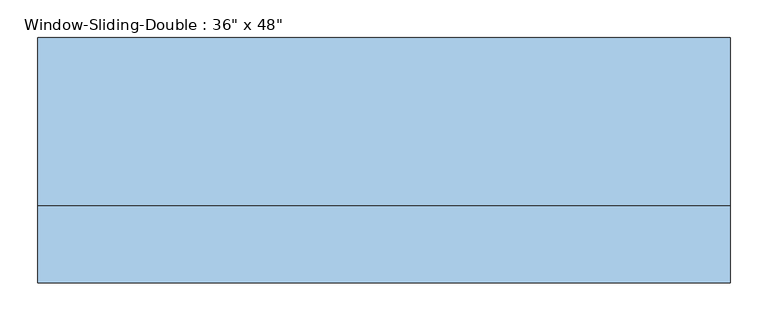
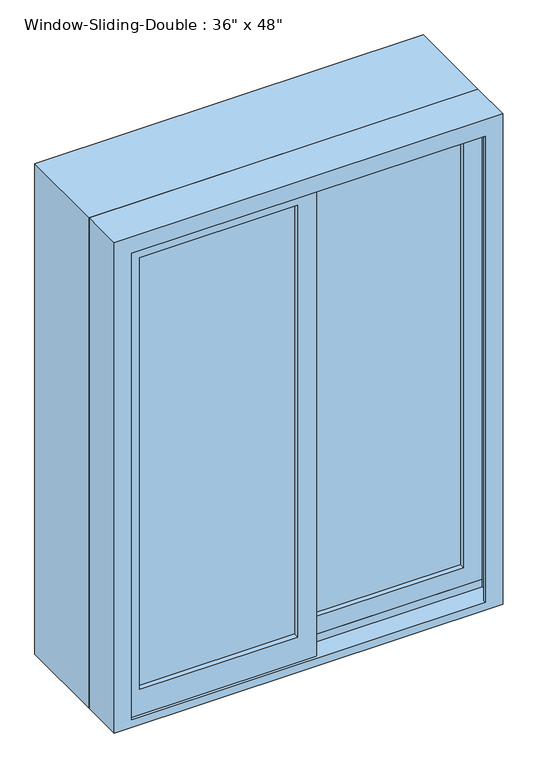
"""IFC4 building model written with IfcOpenShell, lengths in millimetres: window geometry."""

from ifc_helpers import new_model, si_unit, frame, origin, place, context, project, spatial, polyline, outline, extrude, faceted_brep, source, transform, mapped, element, save


def window_970b94cb(model_context):
    return source(origin(), model_context, "Body", "SolidModel", [
        faceted_brep([(-457.2, -66.04, 914.4), (457.2, -66.04, 914.4), (457.2, -167.64, 914.4), (-457.2, -167.64, 914.4), (-416.2778905, -167.64, 2092.6778905), (-416.2778905, -167.64, 933.45), (-416.2778905, -161.29, 933.45), (-416.2778905, -161.29, 2092.6778905), (-438.15, -161.29, 933.45), (-438.15, -161.29, 2114.55), (438.15, -161.29, 2114.55), (438.15, -161.29, 933.45), (416.2778905, -161.29, 933.45), (416.2778905, -161.29, 2092.6778905), (-438.15, -116.84, 933.45), (-438.15, -116.84, 952.5), (-438.15, -72.39, 952.5), (-438.15, -72.39, 933.45), (-438.15, -66.04, 933.45), (-438.15, -66.04, 2114.55), (-457.2, -66.04, 2133.6), (457.2, -66.04, 2133.6), (438.15, -66.04, 2114.55), (438.15, -66.04, 933.45), (-457.2, -167.64, 2133.6), (457.2, -167.64, 2133.6), (416.2778905, -167.64, 2092.6778905), (416.2778905, -167.64, 933.45), (438.15, -72.39, 933.45), (438.15, -72.39, 952.5), (438.15, -116.84, 952.5), (438.15, -116.84, 933.45)], [[[0, 1, 2, 3]], [[4, 5, 6, 7]], [[7, 6, 8, 9, 10, 11, 12, 13]], [[9, 8, 14, 15, 16, 17, 18, 19]], [[0, 20, 21, 1], [22, 19, 18, 23]], [[24, 20, 0, 3]], [[2, 25, 24, 3], [4, 26, 27, 5]], [[7, 13, 26, 4]], [[9, 19, 22, 10]], [[20, 24, 25, 21]], [[13, 12, 27, 26]], [[22, 23, 28, 29, 30, 31, 11, 10]], [[21, 25, 2, 1]], [[27, 12, 11, 31, 14, 8, 6, 5]], [[31, 30, 15, 14]], [[30, 29, 16, 15]], [[29, 28, 17, 16]], [[18, 17, 28, 23]]]),
        extrude(outline(polyline([(2133.6, 457.2), (2133.6, -457.2), (914.4, -457.2), (914.4, 457.2), (2133.6, 457.2)]), holes=[polyline([(2114.55, -438.15), (2114.55, 438.15), (933.45, 438.15), (933.45, -438.15), (2114.55, -438.15)])]), frame((0.0, -66.04, 0.0), z_axis=(0.0, 1.0, 0.0), x_axis=(0.0, 0.0, 1.0)), (0.0, 0.0, 1.0), 222.25),
        extrude(outline(polyline([(393.7, -104.14), (22.225, -104.14), (22.225, -97.79), (393.7, -97.79), (393.7, -104.14)])), frame((0.0, 0.0, 996.95), z_axis=(0.0, 0.0, 1.0), x_axis=(1.0, 0.0, 0.0)), (0.0, 0.0, 1.0), 1073.15),
        extrude(outline(polyline([(393.7, -91.44), (22.225, -91.44), (22.225, -85.09), (393.7, -85.09), (393.7, -91.44)])), frame((0.0, 0.0, 996.95), z_axis=(0.0, 0.0, 1.0), x_axis=(1.0, 0.0, 0.0)), (0.0, 0.0, 1.0), 1073.15),
        extrude(outline(polyline([(-22.225, -148.59), (-393.7, -148.59), (-393.7, -142.24), (-22.225, -142.24), (-22.225, -148.59)])), frame((0.0, 0.0, 996.95), z_axis=(0.0, 0.0, 1.0), x_axis=(1.0, 0.0, 0.0)), (0.0, 0.0, 1.0), 1073.15),
        extrude(outline(polyline([(-22.225, -135.89), (-393.7, -135.89), (-393.7, -129.54), (-22.225, -129.54), (-22.225, -135.89)])), frame((0.0, 0.0, 996.95), z_axis=(0.0, 0.0, 1.0), x_axis=(1.0, 0.0, 0.0)), (0.0, 0.0, 1.0), 1073.15),
        extrude(outline(polyline([(933.45, 22.225), (2114.55, 22.225), (2114.55, -438.15), (933.45, -438.15), (933.45, 22.225)]), holes=[polyline([(2070.1, -393.7), (2070.1, -22.225), (996.95, -22.225), (996.95, -393.7), (2070.1, -393.7)])]), frame((0.0, -161.29, 0.0), z_axis=(0.0, 1.0, 0.0), x_axis=(0.0, 0.0, 1.0)), (0.0, 0.0, 1.0), 44.45),
        extrude(outline(polyline([(952.5, -22.225), (952.5, 438.15), (2114.55, 438.15), (2114.55, -22.225), (952.5, -22.225)]), holes=[polyline([(996.95, 393.7), (996.95, 22.225), (2070.1, 22.225), (2070.1, 393.7), (996.95, 393.7)])]), frame((0.0, -116.84, 0.0), z_axis=(0.0, 1.0, 0.0), x_axis=(0.0, 0.0, 1.0)), (0.0, 0.0, 1.0), 44.45),
    ])


if __name__ == "__main__":
    model = new_model("IFC4")
    model_context = context("Model", 3, world=origin())
    ifc_project = project(units=[si_unit("LENGTHUNIT", "METRE", prefix="MILLI")], contexts=[model_context])
    site = spatial("IfcSite", under=ifc_project)
    building = spatial("IfcBuilding", under=site)
    placement = place(None, origin())
    window_shape = window_970b94cb(model_context)
    element("IfcWindow", 1, ObjectType="Window-Sliding-Double : 36\" x 48\"", at=placement, inside=building, context=model_context, shape_type="MappedRepresentation", body=[
        mapped(window_shape, transform((0.0, 0.0, 0.0), x_axis=(1.0, 0.0, 0.0), y_axis=(0.0, 1.0, 0.0), z_axis=(0.0, 0.0, 1.0))),
    ])
    save(model, "model.ifc")

# Revit data of these elements
# Type "Window-Sliding-Double : 36\" x 48\""
#   Type Mark = "E"
#   Fire Rating = "0.5h"
#   Assembly Code = "B2020100"
#   Analytic Construction = "Double glazing - domestic"
#   Window Inset [instance default] = 0' - 0"
#   Wall Thickness [instance default] = 0' - 6"
#   Visual Light Transmittance = 0.81
#   Thermal Resistance (R) = 1.8146 (h·ft²·°F)/BTU
#   Solar Heat Gain Coefficient = 0.76
#   Muntin Width = 1' - 2 5/8"
#   Muntin Height = 3' - 6 1/4"
#   Interior Wall Closure [instance default] = 0' - 2 3/4"
#   Heat Transfer Coefficient (U) = 0.5511 BTU/(h·ft²·°F)
#   Frame Extension [instance default] = 0' - 0 1/4"
#   Exterior Wall Closure [instance default] = 0' - 1 1/4"
#   Rough Width = 3' - 0 1/2"
#   Rough Height = 4' - 0 1/2"
#   Height = 4' - 0"
#   Extension Jamb [instance default] = 0' - 2 3/4"
#   Default Sill Height = 3' - 0"
#   Width = 3' - 0"
#   Interior Trim Visibility [instance default] = yes
#   Indicator Visibility [instance default] = yes
#   Exterior Trim Visibility [instance default] = yes
#   Muntin Visibility = yes
#   Extension Jamb Visibility [instance default] = yes
#   Muntin Pattern = Muntin Pattern_2x2 : Muntin Pattern_2x2
#   Interior Trim Material = Wood - Stained
#   Interior Trim = Trim-Window-Interior-Flat : Picture Frame
#   Interior Frame Material = Wood - Stained
#   Glass Panel Material = Glass
#   Exterior Trim Material = Clad - White
#   Exterior Trim = Trim-Window-Exterior-Flat : with Sill
#   Exterior Frame Material = Clad - White
#   Wall Closure = (empty or 0)
# Element 1 (IfcWindow, "Window-Sliding-Double : 36\" x 48\"")
#   Wall Thickness = 1' - 0"
#   Extension Jamb = 0' - 8 3/4"
#   Materials on its faces: "Wood - Stained", "Glass", "Clad - White"
# Materials
#   "Wood - Stained": class "Wood", colour RGB 224 178 126, transparency 0, Cost = 0
#   "Glass": class "Unassigned", colour RGB 0 128 192, transparency 0.75, Description = "Glass"
#   "Clad - White": class "Wood", colour RGB 242 242 238, transparency 0, Cost = 0
